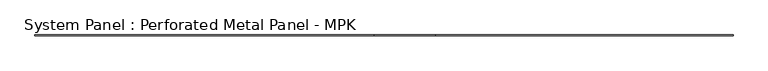
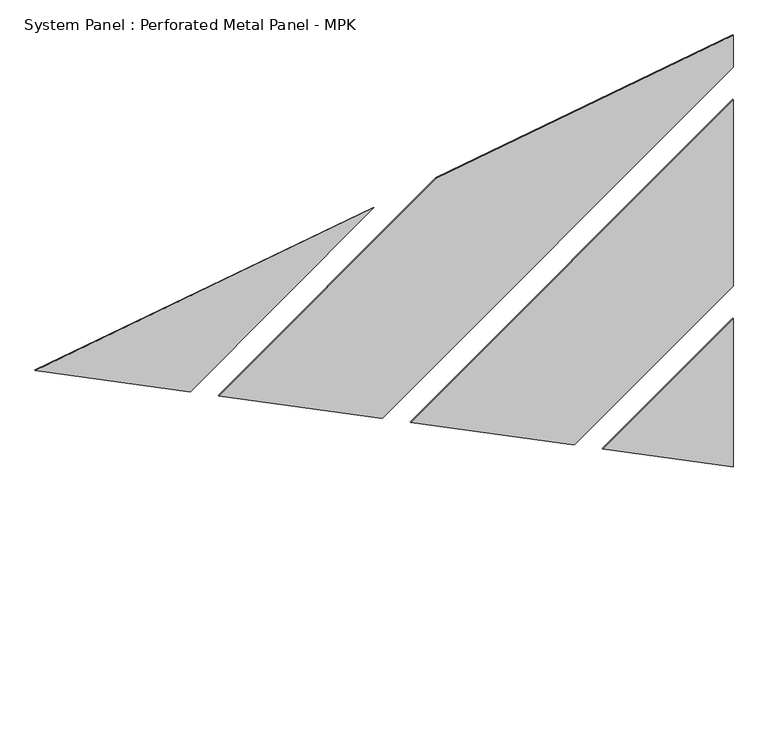
"""IFC4 building model written with IfcOpenShell, lengths in millimetres: plate geometry, System Panel : Perforated Metal Panel - MPK."""

from ifc_helpers import new_model, si_unit, frame, origin, place, context, project, spatial, polyline, outline, extrude, source, transform, mapped, element, save


def system_panel_perforated_metal_panel_mpk_0f825df9(model_context):
    return source(origin(), model_context, "Body", "SweptSolid", [
        extrude(outline(polyline([(11184.6599937, -11269.7002959), (8703.9841202, -6270.6259134), (12913.1936973, -335.4698564), (11184.6599937, -11269.7002959)])), frame((0.0, 0.0, 0.0), z_axis=(0.0, 1.0, 0.0), x_axis=(0.0, 0.0, 1.0)), (0.0, 0.0, 1.0), 20.0),
        extrude(outline(polyline([(2088.4957795, 7060.9498257), (0.0, 11269.7002959), (5073.3394157, 11269.7002959), (2088.4957795, 7060.9498257)])), frame((0.0, 0.0, 0.0), z_axis=(0.0, 1.0, 0.0), x_axis=(0.0, 0.0, 1.0)), (0.0, 0.0, 1.0), 20.0),
        extrude(outline(polyline([(8247.6570135, -5351.0325181), (5624.4035032, -64.6347415), (13662.7079945, 11269.7002959), (14747.7926529, 11269.7002959), (13231.1621962, 1675.9117166), (8247.6570135, -5351.0325181)])), frame((0.0, 0.0, 0.0), z_axis=(0.0, 1.0, 0.0), x_axis=(0.0, 0.0, 1.0)), (0.0, 0.0, 1.0), 20.0),
        extrude(outline(polyline([(5168.0763965, 854.9586538), (2544.8228862, 6141.3564304), (6181.8416783, 11269.7002959), (12554.2057319, 11269.7002959), (5168.0763965, 854.9586538)])), frame((0.0, 0.0, 0.0), z_axis=(0.0, 1.0, 0.0), x_axis=(0.0, 0.0, 1.0)), (0.0, 0.0, 1.0), 20.0),
    ])


if __name__ == "__main__":
    model = new_model("IFC4")
    model_context = context("Model", 3, world=origin())
    ifc_project = project(units=[si_unit("LENGTHUNIT", "METRE", prefix="MILLI")], contexts=[model_context])
    site = spatial("IfcSite", under=ifc_project)
    building = spatial("IfcBuilding", under=site)
    placement = place(None, origin())
    system_panel_perforated_metal_panel_mpk_shape = system_panel_perforated_metal_panel_mpk_0f825df9(model_context)
    element("IfcPlate", 1, ObjectType="System Panel : Perforated Metal Panel - MPK", at=placement, inside=building, context=model_context, shape_type="MappedRepresentation", body=[
        mapped(system_panel_perforated_metal_panel_mpk_shape, transform((0.0, 0.0, 0.0), x_axis=(1.0, 0.0, 0.0), y_axis=(0.0, 1.0, 0.0), z_axis=(0.0, 0.0, 1.0))),
    ])
    save(model, "model.ifc")

# Revit data of these elements
# Element 1 (IfcPlate, "System Panel : Perforated Metal Panel - MPK")
#   Materials on its faces: "Perforated  Metal Panels - MPK"
# Materials
#   "Perforated  Metal Panels - MPK": class "Miscellaneous", colour RGB 127 127 127, transparency 0
